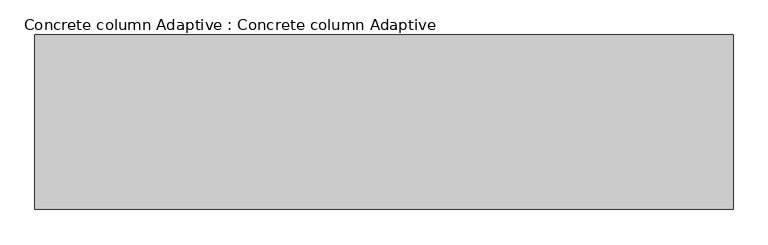
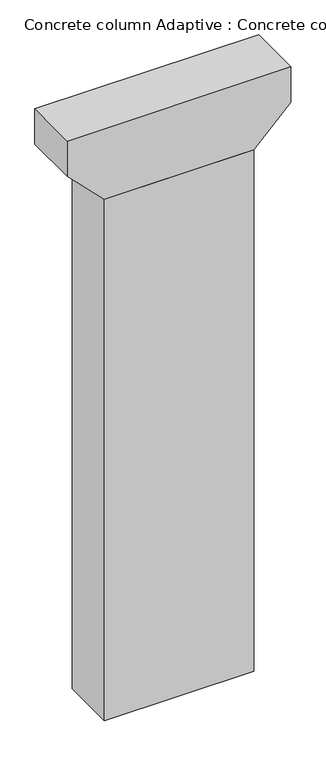
"""IFC4 building model written with IfcOpenShell, lengths in millimetres: proxy geometry, Concrete column Adaptive : Concrete column Adaptive."""

from ifc_helpers import new_model, si_unit, frame, origin, origin_with_axes, place, context, project, spatial, polyline, outline, extrude, source, transform, mapped, element, save


def concrete_column_adaptive_concrete_column_adaptive_048184f4(model_context):
    return source(origin(), model_context, "Body", "SweptSolid", [
        extrude(outline(polyline([(33587.0, 6000.0), (33587.0, -6000.0), (31587.0, -6000.0), (29587.0, -4000.0), (29587.0, 4000.0), (31587.0, 6000.0), (33587.0, 6000.0)])), frame((0.0, -1500.0, 0.0), z_axis=(0.0, 1.0, 0.0), x_axis=(0.0, 0.0, 1.0)), (0.0, 0.0, 1.0), 3000.0),
        extrude(outline(polyline([(-4000.0, -1500.0), (-4000.0, 1500.0), (4000.0, 1500.0), (4000.0, -1500.0), (-4000.0, -1500.0)])), origin_with_axes(), (0.0, 0.0, 1.0), 29587.0),
    ])


if __name__ == "__main__":
    model = new_model("IFC4")
    model_context = context("Model", 3, world=origin())
    ifc_project = project(units=[si_unit("LENGTHUNIT", "METRE", prefix="MILLI")], contexts=[model_context])
    site = spatial("IfcSite", under=ifc_project)
    building = spatial("IfcBuilding", under=site)
    placement = place(None, origin())
    concrete_column_adaptive_concrete_column_adaptive_shape = concrete_column_adaptive_concrete_column_adaptive_048184f4(model_context)
    element("IfcBuildingElementProxy", 1, Name="Concrete column Adaptive : Concrete column Adaptive", ObjectType="Concrete column Adaptive : Concrete column Adaptive", at=placement, inside=building, context=model_context, shape_type="MappedRepresentation", body=[
        mapped(concrete_column_adaptive_concrete_column_adaptive_shape, transform((0.0, 0.0, 0.0), x_axis=(1.0, 0.0, 0.0), y_axis=(0.0, 1.0, 0.0), z_axis=(0.0, 0.0, 1.0))),
    ])
    save(model, "model.ifc")

# Revit data of these elements
# Type "Concrete column Adaptive : Concrete column Adaptive"
#   Height [instance default] = 30000 mm
#   Default Elevation = 0
# Element 1 (IfcBuildingElementProxy, "Concrete column Adaptive : Concrete column Adaptive")
#   Height = 29587 mm
#   Materials on its faces: "Default Wall"
# Materials
#   "Default Wall": class "Miscellaneous", colour RGB 128 128 128, transparency 0, Comments = "Rendering appearance not upgraded Rendering appearance not upgraded ", Cost = 0
